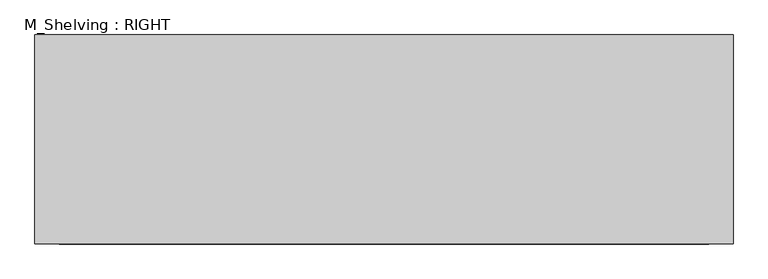
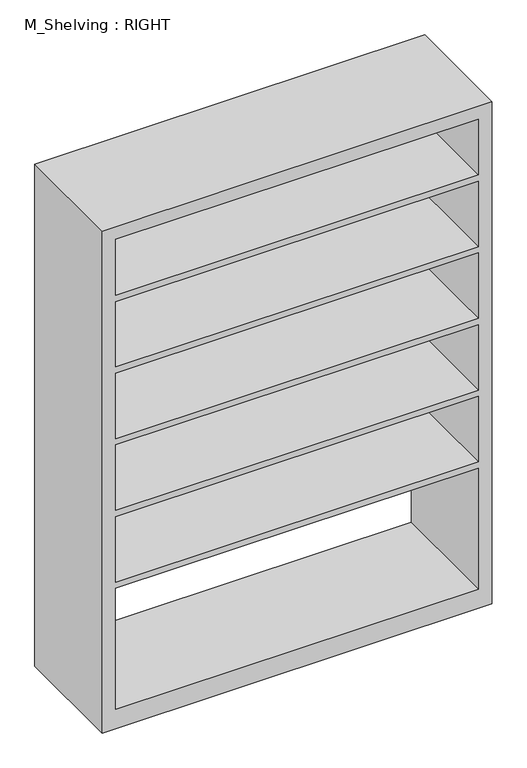
"""IFC4 building model written with IfcOpenShell, lengths in millimetres: furniture geometry, M_Shelving : RIGHT."""

from ifc_helpers import new_model, si_unit, frame, origin, place, context, project, spatial, polyline, outline, extrude, source, transform, mapped, element, save


def m_shelving_right_232c7dd4(model_context):
    return source(origin(), model_context, "Body", "SweptSolid", [
        extrude(outline(polyline([(0.0, 735.0), (2000.0, 735.0), (2000.0, -735.0), (0.0, -735.0), (0.0, 735.0)]), holes=[polyline([(1949.2, 684.2), (1726.9857143, 684.2), (1726.9857143, -684.2), (1949.2, -684.2), (1949.2, 684.2)]), polyline([(76.2, 684.2), (76.2, -684.2), (558.7285714, -684.2), (558.7285714, 684.2), (76.2, 684.2)]), polyline([(1155.5571429, -684.2), (1415.8714286, -684.2), (1415.8714286, 684.2), (1155.5571429, 684.2), (1155.5571429, -684.2)]), polyline([(1701.5857143, 684.2), (1441.2714286, 684.2), (1441.2714286, -684.2), (1701.5857143, -684.2), (1701.5857143, 684.2)]), polyline([(1130.1571429, 684.2), (869.8428571, 684.2), (869.8428571, -684.2), (1130.1571429, -684.2), (1130.1571429, 684.2)]), polyline([(844.4428571, 684.2), (584.1285714, 684.2), (584.1285714, -684.2), (844.4428571, -684.2), (844.4428571, 684.2)])]), frame((0.0, -524.8, 0.0), z_axis=(0.0, 1.0, 0.0), x_axis=(0.0, 0.0, 1.0)), (0.0, 0.0, 1.0), 440.0),
    ])


if __name__ == "__main__":
    model = new_model("IFC4")
    model_context = context("Model", 3, world=origin())
    ifc_project = project(units=[si_unit("LENGTHUNIT", "METRE", prefix="MILLI")], contexts=[model_context])
    site = spatial("IfcSite", under=ifc_project)
    building = spatial("IfcBuilding", under=site)
    placement = place(None, origin())
    m_shelving_right_shape = m_shelving_right_232c7dd4(model_context)
    element("IfcFurniture", 1, ObjectType="M_Shelving : RIGHT", at=placement, inside=building, context=model_context, shape_type="MappedRepresentation", body=[
        mapped(m_shelving_right_shape, transform((0.0, 0.0, 0.0), x_axis=(1.0, 0.0, 0.0), y_axis=(0.0, 1.0, 0.0), z_axis=(0.0, 0.0, 1.0))),
    ])
    save(model, "model.ifc")

# Revit data of these elements
# Type "M_Shelving : RIGHT"
#   Depth = 440 mm
#   Height = 2000 mm
#   Width = 1470 mm
#   Material = Birch
#   Default Elevation = 0
# Element 1 (IfcFurniture, "M_Shelving : RIGHT")
#   Materials on its faces: "Birch"
# Materials
#   "Birch": class "Wood", colour RGB 224 178 126, transparency 0, Description = "Betula Alleghaniensis", Cost = 0
